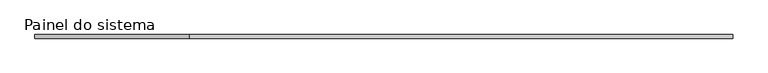
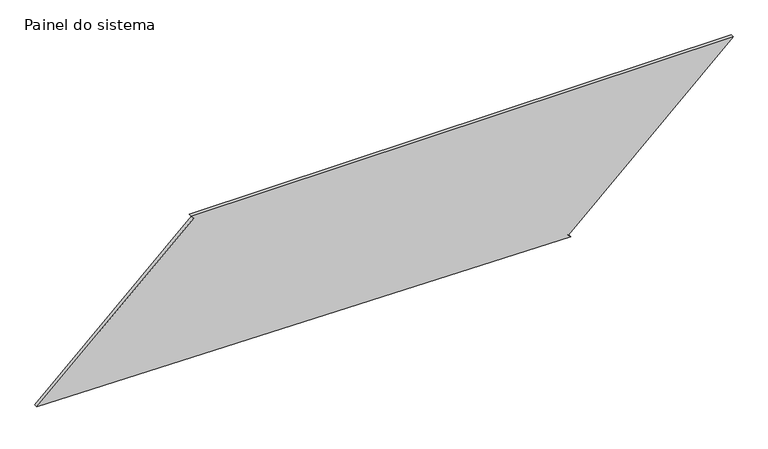
"""IFC4 building model written with IfcOpenShell, lengths in millimetres: plate geometry, Painel do sistema : Envidraçado."""

from ifc_helpers import new_model, si_unit, frame, origin, place, context, project, spatial, polyline, outline, extrude, source, transform, mapped, element, save


def painel_do_sistema_d04ed3bf(model_context):
    return source(origin(), model_context, "Body", "SweptSolid", [
        extrude(outline(polyline([(0.0, 1289.2278592), (18.3764951, 1272.2778024), (1071.6720598, 2414.2138443), (1071.6720598, -1343.3383614), (1053.2955647, -1326.3883045), (49.9102838, -2414.2138443), (0.0, 1289.2278592)])), frame((0.0, 24.5, 0.0), z_axis=(0.0, 1.0, 0.0), x_axis=(0.0, 0.0, 1.0)), (0.0, 0.0, 1.0), 25.0),
    ])


if __name__ == "__main__":
    model = new_model("IFC4")
    model_context = context("Model", 3, world=origin())
    ifc_project = project(units=[si_unit("LENGTHUNIT", "METRE", prefix="MILLI")], contexts=[model_context])
    site = spatial("IfcSite", under=ifc_project)
    building = spatial("IfcBuilding", under=site)
    placement = place(None, origin())
    painel_do_sistema_shape = painel_do_sistema_d04ed3bf(model_context)
    element("IfcPlate", 1, ObjectType="Painel do sistema : Envidraçado", at=placement, inside=building, context=model_context, shape_type="MappedRepresentation", body=[
        mapped(painel_do_sistema_shape, transform((0.0, 0.0, 0.0), x_axis=(1.0, 0.0, 0.0), y_axis=(0.0, 1.0, 0.0), z_axis=(0.0, 0.0, 1.0))),
    ])
    save(model, "model.ifc")

# Revit data of these elements
# Type "Painel do sistema : Envidraçado"
#   Construction Type Id = "GSP4R"
#   Analytic Construction = "Vidraça única Pilkington 1/8 pol"
#   Visual Light Transmittance = 0.9
#   Solar Heat Gain Coefficient = 0.86
#   Heat Transfer Coefficient (U) = 6.7069 W/(m²·K)
# Element 1 (IfcPlate, "Painel do sistema : Envidraçado")
#   Materials on its faces: "Vidro"
# Materials
#   "Vidro": class "Vidro", colour RGB 0 128 192, transparency 0.9, Description = "Vidro de sílica", Cost = 0
